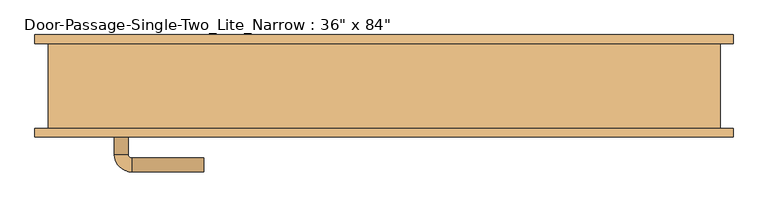
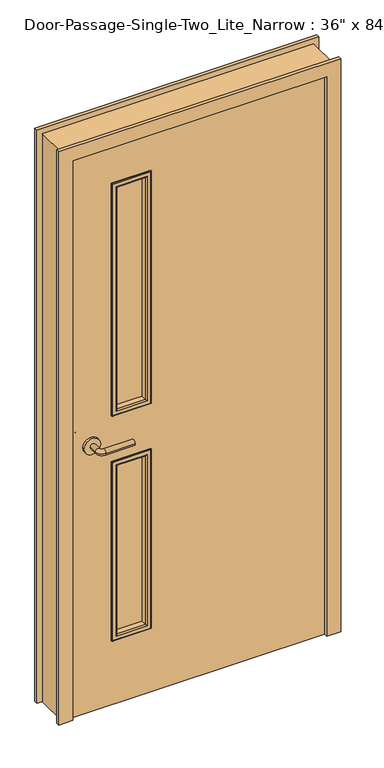
"""IFC4 building model written with IfcOpenShell, lengths in millimetres: door geometry."""

import ifcopenshell
import ifcopenshell.guid

model = None  # the IFC model being written
_history = None  # IfcOwnerHistory: only IFC2X3 demands one
_inside = {}  # id of a spatial element -> (the spatial element, [elements in it])
_under = {}  # id of a project, library or spatial element -> (it, [spatial elements below it])
_declared = {}  # id of a project -> (the project, [libraries it declares])
_typed = {}  # id of a type object -> (the type object, [elements of that type])
_made_of = {}  # id of a material, layer set ... -> (it, [elements and type objects made of it])


def new_model(schema):
    """Start an empty IFC model of exactly this schema.

    Asked for "IFC4X3", IfcOpenShell would pick the latest addendum, in which some entities
    have other attributes; the version numbers below select the first issue.
    IFC2X3 requires an IfcOwnerHistory on every rooted entity: one is made here for all.
    """
    global model, _history
    if schema == "IFC4X3":
        model = ifcopenshell.file(schema_version=(4, 3, 0, 0))
    else:
        model = ifcopenshell.file(schema=schema)
    _inside.clear()
    _under.clear()
    _declared.clear()
    _typed.clear()
    _made_of.clear()
    _history = None
    if model.schema == "IFC2X3":
        org = make("IfcOrganization", Name="unknown")
        user = make(
            "IfcPersonAndOrganization",
            ThePerson=make("IfcPerson", FamilyName="unknown"),
            TheOrganization=org,
        )
        app = make(
            "IfcApplication",
            ApplicationDeveloper=org,
            Version="unknown",
            ApplicationFullName="unknown",
            ApplicationIdentifier="unknown",
        )
        _history = make(
            "IfcOwnerHistory",
            OwningUser=user,
            OwningApplication=app,
            ChangeAction="ADDED",
            CreationDate=0,
        )
    return model


def make(cls, **values):
    """One entity of the class cls with the attributes given. An attribute that is None is left unset."""
    return model.create_entity(
        cls, **{name: value for name, value in values.items() if value is not None}
    )


def rooted(cls, **values):
    """An entity with a GlobalId (a new one), such as an element, a storey or a relation."""
    return make(cls, GlobalId=ifcopenshell.guid.new(), OwnerHistory=_history, **values)


def si_unit(unit_type, name, prefix=None):
    """IfcSIUnit, for example si_unit("LENGTHUNIT", "METRE", prefix="MILLI")."""
    return make("IfcSIUnit", UnitType=unit_type, Prefix=prefix, Name=name)


def assignment(units):
    """IfcUnitAssignment: the units of a project."""
    return None if units is None else make("IfcUnitAssignment", Units=units)


def point(xyz):
    """IfcCartesianPoint."""
    return None if xyz is None else make("IfcCartesianPoint", Coordinates=xyz)


def direction(xyz):
    """IfcDirection."""
    return None if xyz is None else make("IfcDirection", DirectionRatios=xyz)


def frame(location, z_axis=None, x_axis=None):
    """IfcAxis2Placement3D, a coordinate frame: its origin and axes. An axis left out is left unset."""
    return make(
        "IfcAxis2Placement3D",
        Location=point(location),
        Axis=direction(z_axis),
        RefDirection=direction(x_axis),
    )


def frame_2d(location, x_axis=None):
    """IfcAxis2Placement2D, a coordinate frame in the plane: its origin and x axis."""
    return make(
        "IfcAxis2Placement2D", Location=point(location), RefDirection=direction(x_axis)
    )


def origin():
    """The frame at (0, 0, 0) with its axes left unset."""
    return frame((0.0, 0.0, 0.0))


def place(relative_to, where):
    """IfcLocalPlacement: puts the frame where relative to a parent placement (None: the world)."""
    return make(
        "IfcLocalPlacement", PlacementRelTo=relative_to, RelativePlacement=where
    )


def context(
    kind, dimensions, precision=None, world=None, true_north=None, identifier=None
):
    """IfcGeometricRepresentationContext, for example the 3D "Model" context."""
    return make(
        "IfcGeometricRepresentationContext",
        ContextIdentifier=identifier,
        ContextType=kind,
        CoordinateSpaceDimension=dimensions,
        Precision=precision,
        WorldCoordinateSystem=world,
        TrueNorth=true_north,
    )


def project(units=None, contexts=None):
    """IfcProject with its units and contexts."""
    return rooted(
        "IfcProject",
        Name="project",
        RepresentationContexts=contexts,
        UnitsInContext=assignment(units),
    )


def spatial(cls, under=None, at=None, **own):
    """A site, building, storey or space (cls), placed at a placement, below another one or the project."""
    s = rooted(cls, ObjectPlacement=at, **own)
    if under is not None:
        _under.setdefault(under.id(), (under, []))[1].append(s)
    return s


def polyline(points):
    """IfcPolyline through the points."""
    return make("IfcPolyline", Points=[point(p) for p in points])


def circle_curve(where, radius):
    """IfcCircle in the frame where."""
    return make("IfcCircle", Position=where, Radius=radius)


def ellipse_curve(where, semi_axis1, semi_axis2):
    """IfcEllipse in the frame where."""
    return make(
        "IfcEllipse", Position=where, SemiAxis1=semi_axis1, SemiAxis2=semi_axis2
    )


def trimmed(basis, trim1, trim2, sense, master):
    """IfcTrimmedCurve: the piece of a basis curve between two trims."""
    return make(
        "IfcTrimmedCurve",
        BasisCurve=basis,
        Trim1=trim1,
        Trim2=trim2,
        SenseAgreement=sense,
        MasterRepresentation=master,
    )


def segment(curve, same_sense, transition):
    """IfcCompositeCurveSegment."""
    return make(
        "IfcCompositeCurveSegment",
        Transition=transition,
        SameSense=same_sense,
        ParentCurve=curve,
    )


def composite_curve(segments, self_intersect=None):
    """IfcCompositeCurve: segments joined end to end."""
    return make("IfcCompositeCurve", Segments=segments, SelfIntersect=self_intersect)


def outline(outer, holes=None, kind="AREA"):
    """IfcArbitraryClosedProfileDef: a profile drawn as a closed curve; with holes, ...WithVoids."""
    if holes is None:
        return make("IfcArbitraryClosedProfileDef", ProfileType=kind, OuterCurve=outer)
    return make(
        "IfcArbitraryProfileDefWithVoids",
        ProfileType=kind,
        OuterCurve=outer,
        InnerCurves=holes,
    )


def extrude(swept, where, along, depth):
    """IfcExtrudedAreaSolid: the profile swept, set in the frame where, extruded along a direction by depth."""
    return make(
        "IfcExtrudedAreaSolid",
        SweptArea=swept,
        Position=where,
        ExtrudedDirection=direction(along),
        Depth=depth,
    )


def faces_of(points, faces, orient=None, outer=None):
    """IfcFace entities. A face is a list of loops; a loop is a list of indices into points, from 0.

    orient and outer hold one flag for each loop. By default every Orientation is true, the
    first loop of a face is its IfcFaceOuterBound and the others are IfcFaceBound.
    """
    made = []
    for i, loops in enumerate(faces):
        bounds = []
        for j, loop in enumerate(loops):
            is_outer = j == 0 if outer is None else outer[i][j]
            bounds.append(
                make(
                    "IfcFaceOuterBound" if is_outer else "IfcFaceBound",
                    Bound=make("IfcPolyLoop", Polygon=[points[k] for k in loop]),
                    Orientation=True if orient is None else orient[i][j],
                )
            )
        made.append(make("IfcFace", Bounds=bounds))
    return made


def faceted_brep(points, faces, orient=None, outer=None, voids=None):
    """IfcFacetedBrep: a solid bounded by flat faces; with voids (closed shells), ...WithVoids."""
    shared = [point(p) for p in points]
    hull = make("IfcClosedShell", CfsFaces=faces_of(shared, faces, orient, outer))
    if voids is None:
        return make("IfcFacetedBrep", Outer=hull)
    return make(
        "IfcFacetedBrepWithVoids",
        Outer=hull,
        Voids=[
            make(cls, CfsFaces=faces_of(shared, fs, o, b)) for cls, fs, o, b in voids
        ],
    )


def shape(context_of_items, identifier, shape_type, items):
    """IfcShapeRepresentation: the items that make up one representation, for example the "Body"."""
    return make(
        "IfcShapeRepresentation",
        ContextOfItems=context_of_items,
        RepresentationIdentifier=identifier,
        RepresentationType=shape_type,
        Items=items,
    )


def source(mapping_origin, context_of_items, identifier, shape_type, items):
    """IfcRepresentationMap: a shape defined once, which mapped items show again and again."""
    return make(
        "IfcRepresentationMap",
        MappingOrigin=mapping_origin,
        MappedRepresentation=shape(context_of_items, identifier, shape_type, items),
    )


def transform(
    local_origin,
    x_axis=None,
    y_axis=None,
    z_axis=None,
    scale=None,
    scale2=None,
    scale3=None,
    uniform=True,
):
    """IfcCartesianTransformationOperator3D, or its non-uniform kind. x_axis, y_axis, z_axis: its Axis1, 2, 3."""
    if uniform:
        return make(
            "IfcCartesianTransformationOperator3D",
            Axis1=direction(x_axis),
            Axis2=direction(y_axis),
            LocalOrigin=point(local_origin),
            Scale=scale,
            Axis3=direction(z_axis),
        )
    return make(
        "IfcCartesianTransformationOperator3DnonUniform",
        Axis1=direction(x_axis),
        Axis2=direction(y_axis),
        LocalOrigin=point(local_origin),
        Scale=scale,
        Axis3=direction(z_axis),
        Scale2=scale2,
        Scale3=scale3,
    )


def mapped(mapping_source, mapping_target):
    """IfcMappedItem: shows the shape of a source again, moved by a transform."""
    return make(
        "IfcMappedItem", MappingSource=mapping_source, MappingTarget=mapping_target
    )


def made_of(thing, what):
    """Note that an element or type object is made of a material, layer set ...; save() writes the relation."""
    if what is not None:
        _made_of.setdefault(what.id(), (what, []))[1].append(thing)
    return thing


def element(
    cls,
    number,
    at=None,
    inside=None,
    cuts=None,
    type_object=None,
    material=None,
    context=None,
    identifier="Body",
    shape_type=None,
    held_by="IfcProductDefinitionShape",
    body=None,
    shapes=None,
    **own,
):
    """One element of the class cls, such as IfcWall. Its Tag is "e" and its number.

    at: its placement. inside: the storey or other place that contains it. cuts: it is an
    opening in that element (IfcRelVoidsElement). A single representation is given by context,
    identifier, shape_type and body (its items); several are given by shapes. held_by: the class
    of the entity that holds the representations. save() writes the other relations.
    """
    e = rooted(cls, Tag="e%d" % number, ObjectPlacement=at, **own)
    if body is not None:
        shapes = [shape(context, identifier, shape_type, body)]
    if shapes is not None:
        e.Representation = make(held_by, Representations=shapes)
    if inside is not None:
        _inside.setdefault(inside.id(), (inside, []))[1].append(e)
    if cuts is not None:
        rooted(
            "IfcRelVoidsElement", RelatingBuildingElement=cuts, RelatedOpeningElement=e
        )
    if type_object is not None:
        _typed.setdefault(type_object.id(), (type_object, []))[1].append(e)
    return made_of(e, material)


def aggregate(whole, parts):
    """IfcRelAggregates: a whole, such as a stair, and the parts it consists of."""
    return rooted("IfcRelAggregates", RelatingObject=whole, RelatedObjects=parts)


def save(model, path):
    """Write the relations noted so far, then the file.

    IfcRelAggregates (storeys below a building ...), IfcRelContainedInSpatialStructure (elements
    in a storey), IfcRelDefinesByType, IfcRelAssociatesMaterial and IfcRelDeclares: one each for
    every whole, place, type object, material and project.
    """
    for whole, parts in _under.values():
        aggregate(whole, parts)
    for where, things in _inside.values():
        rooted(
            "IfcRelContainedInSpatialStructure",
            RelatedElements=things,
            RelatingStructure=where,
        )
    for kind, things in _typed.values():
        rooted("IfcRelDefinesByType", RelatedObjects=things, RelatingType=kind)
    for what, things in _made_of.values():
        rooted("IfcRelAssociatesMaterial", RelatedObjects=things, RelatingMaterial=what)
    for by, libraries in _declared.values():
        rooted("IfcRelDeclares", RelatingContext=by, RelatedDefinitions=libraries)
    model.write(path)


def plane_surface(at):
    """IfcPlane: the flat surface through the origin of the frame at, square to its z axis."""
    return make("IfcPlane", Position=at)


def cylinder_surface(at, radius):
    """IfcCylindricalSurface: all points at the distance radius from the z axis of the frame at."""
    return make("IfcCylindricalSurface", Position=at, Radius=radius)


def revolved_surface(curve, axis_point, axis_direction):
    """IfcSurfaceOfRevolution: the curve turned about the line through axis_point along axis_direction."""
    return make(
        "IfcSurfaceOfRevolution",
        SweptCurve=make("IfcArbitraryOpenProfileDef", ProfileType="CURVE", Curve=curve),
        AxisPosition=make("IfcAxis1Placement", Location=point(axis_point), Axis=direction(axis_direction)),
    )


def advanced_brep(points, edges, surfaces, faces):
    """IfcAdvancedBrep: a solid bounded by faces that lie on surfaces and meet in shared edges.

    An edge is (start, end): straight between two places in points (the first is 0);
    or (start, end, curve); or (start, end, curve, False) where it runs against its curve.
    A face is (place in surfaces, loops), or (place, loops, False) where it looks against
    its surface's normal. A loop lists edges by number (the first is 1), with a minus sign
    where the edge is run from its end to its start. The first loop is the outer one.
    """
    corners = [point(p) for p in points]
    vertices = [make("IfcVertexPoint", VertexGeometry=c) for c in corners]
    made = []
    for start, end, *more in edges:
        made.append(
            make(
                "IfcEdgeCurve",
                EdgeStart=vertices[start],
                EdgeEnd=vertices[end],
                EdgeGeometry=more[0] if more else make("IfcPolyline", Points=[corners[start], corners[end]]),
                SameSense=more[1] if len(more) > 1 else True,
            )
        )
    hull = []
    for where, loops, *sense in faces:
        bounds = []
        for j, loop in enumerate(loops):
            ring = [make("IfcOrientedEdge", EdgeElement=made[abs(k) - 1], Orientation=k > 0) for k in loop]
            bounds.append(
                make(
                    "IfcFaceOuterBound" if j == 0 else "IfcFaceBound",
                    Bound=make("IfcEdgeLoop", EdgeList=ring),
                    Orientation=True,
                )
            )
        hull.append(make("IfcAdvancedFace", Bounds=bounds, FaceSurface=surfaces[where], SameSense=sense[0] if sense else True))
    return make("IfcAdvancedBrep", Outer=make("IfcClosedShell", CfsFaces=hull))


def door_7eef6684(model_context):
    return source(origin(), model_context, "Body", "SolidModel", [
        advanced_brep(
        [(-392.190625, -15.8125, 1016.0), (-372.190625, -15.8125, 1016.0), (-392.190625, 14.1875, 1016.0), (-372.190625, 14.1875, 1016.0), (-367.190625, 19.1875, 1016.0), (-367.190625, 39.1875, 1016.0), (-262.190625, 39.1875, 1016.0), (-262.190625, 19.1875, 1016.0)],
        [
            (0, 1, circle_curve(frame((-382.190625, -15.8125, 1016.0), z_axis=(0.0, -1.0, 0.0), x_axis=(1.0, 0.0, 0.0)), 10.0)),
            (1, 0, circle_curve(frame((-382.190625, -15.8125, 1016.0), z_axis=(0.0, -1.0, 0.0), x_axis=(1.0, 0.0, 0.0)), 10.0)),
            (0, 2),
            (2, 3, circle_curve(frame((-382.190625, 14.1875, 1016.0), z_axis=(0.0, -1.0, 0.0), x_axis=(1.0, 0.0, 0.0)), 10.0)),
            (3, 1),
            (3, 2, circle_curve(frame((-382.190625, 14.1875, 1016.0), z_axis=(0.0, -1.0, 0.0), x_axis=(1.0, 0.0, 0.0)), 10.0)),
            (4, 3, circle_curve(frame((-367.190625, 14.1875, 1016.0), z_axis=(0.0, 0.0, 1.0), x_axis=(-1.0, 0.0, 0.0)), 5.0)),
            (2, 5, circle_curve(frame((-367.190625, 14.1875, 1016.0), z_axis=(0.0, 0.0, -1.0), x_axis=(-1.0, 0.0, 0.0)), 25.0)),
            (5, 4, circle_curve(frame((-367.190625, 29.1875, 1016.0), z_axis=(-1.0, 0.0, 0.0), x_axis=(0.0, -1.0, 0.0)), 10.0)),
            (4, 5, circle_curve(frame((-367.190625, 29.1875, 1016.0), z_axis=(-1.0, 0.0, 0.0), x_axis=(0.0, -1.0, 0.0)), 10.0)),
            (6, 7, circle_curve(frame((-262.190625, 29.1875, 1016.0), z_axis=(1.0, 0.0, 0.0), x_axis=(0.0, -1.0, 0.0)), 10.0)),
            (7, 6, circle_curve(frame((-262.190625, 29.1875, 1016.0), z_axis=(1.0, 0.0, 0.0), x_axis=(0.0, -1.0, 0.0)), 10.0)),
            (5, 6),
            (7, 4),
        ],
        [
            plane_surface(frame((-382.190625, -15.8125, 1016.0), z_axis=(0.0, -1.0, 0.0), x_axis=(0.0, 0.0, 1.0))),
            cylinder_surface(frame((-382.190625, -15.8125, 1016.0), z_axis=(0.0, -1.0, 0.0), x_axis=(1.0, 0.0, 0.0)), 10.0),
            revolved_surface(trimmed(ellipse_curve(frame((-382.190625, 14.1875, 1016.0), z_axis=(0.0, -1.0, 0.0), x_axis=(1.0, 0.0, 0.0)), 10.0, 10.0), [point((-392.190625, 14.1875, 1016.0))], [point((-372.190625, 14.1875, 1016.0))], True, "CARTESIAN"), (-367.190625, 14.1875, 1016.0), (0.0, 0.0, -1.0)),
            revolved_surface(trimmed(ellipse_curve(frame((-382.190625, 14.1875, 1016.0), z_axis=(0.0, -1.0, 0.0), x_axis=(1.0, 0.0, 0.0)), 10.0, 10.0), [point((-372.190625, 14.1875, 1016.0))], [point((-392.190625, 14.1875, 1016.0))], True, "CARTESIAN"), (-367.190625, 14.1875, 1016.0), (0.0, 0.0, -1.0)),
            plane_surface(frame((-262.190625, 29.1875, 1016.0), z_axis=(1.0, 0.0, 0.0), x_axis=(0.0, 0.0, 1.0))),
            cylinder_surface(frame((-367.190625, 29.1875, 1016.0), z_axis=(-1.0, 0.0, 0.0), x_axis=(0.0, -1.0, 0.0)), 10.0),
        ],
        [
            (0, [[1, 2]]),
            (1, [[-1, 3, 4, 5]]),
            (1, [[-2, -5, 6, -3]]),
            (2, [[7, -4, 8, 9]]),
            (3, [[-8, -6, -7, 10]]),
            (4, [[11, 12]]),
            (5, [[-9, 13, -12, 14]]),
            (5, [[-10, -14, -11, -13]]),
        ],
    ),
        extrude(outline(composite_curve([segment(trimmed(circle_curve(frame_2d((1016.0, -384.690625)), 30.0), [point((1016.0, -414.690625))], [point((1016.0, -354.690625))], False, "CARTESIAN"), True, "CONTINUOUS"), segment(trimmed(circle_curve(frame_2d((1016.0, -384.690625)), 30.0), [point((1016.0, -354.690625))], [point((1016.0, -414.690625))], False, "CARTESIAN"), True, "CONTINUOUS")], self_intersect=False)), frame((0.0, -23.8125, 0.0), z_axis=(0.0, 1.0, 0.0), x_axis=(0.0, 0.0, 1.0)), (0.0, 0.0, 1.0), 8.0),
        advanced_brep(
        [(-392.190625, -76.2625, 1016.0), (-372.190625, -76.2625, 1016.0), (-372.190625, -106.2625, 1016.0), (-392.190625, -106.2625, 1016.0), (-367.190625, -111.2625, 1016.0), (-367.190625, -131.2625, 1016.0), (-262.190625, -131.2625, 1016.0), (-262.190625, -111.2625, 1016.0)],
        [
            (0, 1, circle_curve(frame((-382.190625, -76.2625, 1016.0), z_axis=(0.0, 1.0, 0.0), x_axis=(1.0, 0.0, 0.0)), 10.0)),
            (1, 0, circle_curve(frame((-382.190625, -76.2625, 1016.0), z_axis=(0.0, 1.0, 0.0), x_axis=(1.0, 0.0, 0.0)), 10.0)),
            (1, 2),
            (2, 3, circle_curve(frame((-382.190625, -106.2625, 1016.0), z_axis=(0.0, 1.0, 0.0), x_axis=(1.0, 0.0, 0.0)), 10.0)),
            (3, 0),
            (3, 2, circle_curve(frame((-382.190625, -106.2625, 1016.0), z_axis=(0.0, 1.0, 0.0), x_axis=(1.0, 0.0, 0.0)), 10.0)),
            (4, 5, circle_curve(frame((-367.190625, -121.2625, 1016.0), z_axis=(-1.0, 0.0, 0.0), x_axis=(0.0, 1.0, 0.0)), 10.0)),
            (5, 3, circle_curve(frame((-367.190625, -106.2625, 1016.0), z_axis=(0.0, 0.0, -1.0), x_axis=(-1.0, 0.0, 0.0)), 25.0)),
            (2, 4, circle_curve(frame((-367.190625, -106.2625, 1016.0), z_axis=(0.0, 0.0, 1.0), x_axis=(-1.0, 0.0, 0.0)), 5.0)),
            (5, 4, circle_curve(frame((-367.190625, -121.2625, 1016.0), z_axis=(-1.0, 0.0, 0.0), x_axis=(0.0, 1.0, 0.0)), 10.0)),
            (6, 7, circle_curve(frame((-262.190625, -121.2625, 1016.0), z_axis=(1.0, 0.0, 0.0), x_axis=(0.0, 1.0, 0.0)), 10.0)),
            (7, 6, circle_curve(frame((-262.190625, -121.2625, 1016.0), z_axis=(1.0, 0.0, 0.0), x_axis=(0.0, 1.0, 0.0)), 10.0)),
            (4, 7),
            (6, 5),
        ],
        [
            plane_surface(frame((-382.190625, -76.2625, 1016.0), z_axis=(0.0, 1.0, 0.0), x_axis=(0.0, 0.0, 1.0))),
            cylinder_surface(frame((-382.190625, -76.2625, 1016.0), z_axis=(0.0, 1.0, 0.0), x_axis=(1.0, 0.0, 0.0)), 10.0),
            revolved_surface(trimmed(ellipse_curve(frame((-382.190625, -106.2625, 1016.0), z_axis=(0.0, -1.0, 0.0), x_axis=(1.0, 0.0, 0.0)), 10.0, 10.0), [point((-392.190625, -106.2625, 1016.0))], [point((-372.190625, -106.2625, 1016.0))], True, "CARTESIAN"), (-367.190625, -106.2625, 1016.0), (0.0, 0.0, -1.0)),
            revolved_surface(trimmed(ellipse_curve(frame((-382.190625, -106.2625, 1016.0), z_axis=(0.0, -1.0, 0.0), x_axis=(1.0, 0.0, 0.0)), 10.0, 10.0), [point((-372.190625, -106.2625, 1016.0))], [point((-392.190625, -106.2625, 1016.0))], True, "CARTESIAN"), (-367.190625, -106.2625, 1016.0), (0.0, 0.0, -1.0)),
            plane_surface(frame((-262.190625, -121.2625, 1016.0), z_axis=(1.0, 0.0, 0.0), x_axis=(0.0, 0.0, 1.0))),
            cylinder_surface(frame((-367.190625, -121.2625, 1016.0), z_axis=(-1.0, 0.0, 0.0), x_axis=(0.0, 1.0, 0.0)), 10.0),
        ],
        [
            (0, [[1, 2]]),
            (1, [[3, 4, 5, -2]]),
            (1, [[-5, 6, -3, -1]]),
            (2, [[7, 8, -4, 9]]),
            (3, [[10, -9, -6, -8]]),
            (4, [[11, 12]]),
            (5, [[13, -11, 14, -7]]),
            (5, [[-14, -12, -13, -10]]),
        ],
    ),
        extrude(outline(composite_curve([segment(trimmed(circle_curve(frame_2d((1016.0, -384.690625)), 30.0), [point((1016.0, -414.690625))], [point((1016.0, -354.690625))], False, "CARTESIAN"), True, "CONTINUOUS"), segment(trimmed(circle_curve(frame_2d((1016.0, -384.690625)), 30.0), [point((1016.0, -354.690625))], [point((1016.0, -414.690625))], False, "CARTESIAN"), True, "CONTINUOUS")], self_intersect=False)), frame((0.0, -76.2625, 0.0), z_axis=(0.0, 1.0, 0.0), x_axis=(0.0, 0.0, 1.0)), (0.0, 0.0, 1.0), 8.0),
        faceted_brep([(457.2, -80.9625, 0.0), (457.2, -19.05, 0.0), (441.325, -19.05, 0.0), (441.325, 19.05, 0.0), (457.2, 19.05, 0.0), (457.2, 68.2625, 0.0), (508.0, 68.2625, 0.0), (508.0, 55.5625, 0.0), (488.95, 55.5625, 0.0), (488.95, -68.2625, 0.0), (508.0, -68.2625, 0.0), (508.0, -80.9625, 0.0), (508.0, -80.9625, 2184.4), (-508.0, -80.9625, 2184.4), (-508.0, -80.9625, 0.0), (-457.2, -80.9625, 0.0), (-457.2, -80.9625, 2133.6), (457.2, -80.9625, 2133.6), (508.0, -68.2625, 2184.4), (488.95, -68.2625, 2165.35), (-488.95, -68.2625, 2165.35), (-488.95, -68.2625, 0.0), (-508.0, -68.2625, 0.0), (-508.0, -68.2625, 2184.4), (488.95, 55.5625, 2165.35), (508.0, 55.5625, 2184.4), (-508.0, 55.5625, 2184.4), (-508.0, 55.5625, 0.0), (-488.95, 55.5625, 0.0), (-488.95, 55.5625, 2165.35), (508.0, 68.2625, 2184.4), (457.2, 68.2625, 2133.6), (-457.2, 68.2625, 2133.6), (-457.2, 68.2625, 0.0), (-508.0, 68.2625, 0.0), (-508.0, 68.2625, 2184.4), (457.2, 19.05, 2133.6), (441.325, 19.05, 2117.725), (-441.325, 19.05, 2117.725), (-441.325, 19.05, 0.0), (-457.2, 19.05, 0.0), (-457.2, 19.05, 2133.6), (441.325, -19.05, 2117.725), (457.2, -19.05, 2133.6), (-457.2, -19.05, 2133.6), (-457.2, -19.05, 0.0), (-441.325, -19.05, 0.0), (-441.325, -19.05, 2117.725)], [[[0, 1, 2, 3, 4, 5, 6, 7, 8, 9, 10, 11]], [[11, 12, 13, 14, 15, 16, 17, 0]], [[10, 18, 12, 11]], [[9, 19, 20, 21, 22, 23, 18, 10]], [[8, 24, 19, 9]], [[7, 25, 26, 27, 28, 29, 24, 8]], [[6, 30, 25, 7]], [[5, 31, 32, 33, 34, 35, 30, 6]], [[4, 36, 31, 5]], [[3, 37, 38, 39, 40, 41, 36, 4]], [[2, 42, 37, 3]], [[1, 43, 44, 45, 46, 47, 42, 2]], [[0, 17, 43, 1]], [[18, 23, 13, 12]], [[24, 29, 20, 19]], [[30, 35, 26, 25]], [[36, 41, 32, 31]], [[42, 47, 38, 37]], [[17, 16, 44, 43]], [[15, 14, 22, 21, 28, 27, 34, 33, 40, 39, 46, 45]], [[23, 22, 14, 13]], [[29, 28, 21, 20]], [[35, 34, 27, 26]], [[41, 40, 33, 32]], [[47, 46, 39, 38]], [[16, 15, 45, 44]]]),
        extrude(outline(polyline([(2133.6, -457.2), (0.0, -457.2), (0.0, 457.2), (2133.6, 457.2), (2133.6, -457.2)]), holes=[polyline([(1981.2, -304.8), (1981.2, -177.8), (1111.25, -177.8), (1111.25, -304.8), (1981.2, -304.8)]), polyline([(920.75, -304.8), (920.75, -177.8), (254.0, -177.8), (254.0, -304.8), (920.75, -304.8)])]), frame((0.0, -68.2625, 0.0), z_axis=(0.0, 1.0, 0.0), x_axis=(0.0, 0.0, 1.0)), (0.0, 0.0, 1.0), 44.45),
        extrude(outline(polyline([(-177.8, -42.8625), (-177.8, -49.2125), (-304.8, -49.2125), (-304.8, -42.8625), (-177.8, -42.8625)])), frame((0.0, 0.0, 1111.25), z_axis=(0.0, 0.0, 1.0), x_axis=(1.0, 0.0, 0.0)), (0.0, 0.0, 1.0), 869.95),
        extrude(outline(polyline([(-177.8, -42.8625), (-177.8, -49.2125), (-304.8, -49.2125), (-304.8, -42.8625), (-177.8, -42.8625)])), frame((0.0, 0.0, 254.0), z_axis=(0.0, 0.0, 1.0), x_axis=(1.0, 0.0, 0.0)), (0.0, 0.0, 1.0), 666.75),
        advanced_brep(
        [(-177.8, -42.8625, 920.75), (-177.8, -42.8625, 254.0), (-177.8, -23.8125, 254.0), (-177.8, -23.8125, 920.75), (-189.8, -22.8125, 908.75), (-189.8, -22.8125, 266.0), (-189.8, -42.8625, 266.0), (-189.8, -42.8625, 908.75), (-184.8, -17.8125, 913.75), (-184.8, -17.8125, 261.0), (-169.8, -19.8125, 928.75), (-169.8, -19.8125, 246.0), (-171.8, -17.8125, 248.0), (-171.8, -17.8125, 926.75), (-169.8, -23.8125, 928.75), (-169.8, -23.8125, 246.0), (-304.8, -42.8625, 254.0), (-304.8, -23.8125, 254.0), (-292.8, -22.8125, 266.0), (-292.8, -42.8625, 266.0), (-297.8, -17.8125, 261.0), (-312.8, -19.8125, 246.0), (-310.8, -17.8125, 248.0), (-312.8, -23.8125, 246.0), (-304.8, -42.8625, 920.75), (-304.8, -23.8125, 920.75), (-292.8, -22.8125, 908.75), (-292.8, -42.8625, 908.75), (-297.8, -17.8125, 913.75), (-312.8, -19.8125, 928.75), (-310.8, -17.8125, 926.75), (-312.8, -23.8125, 928.75)],
        [
            (0, 1),
            (1, 2),
            (2, 3),
            (3, 0),
            (4, 5),
            (5, 6),
            (6, 7),
            (7, 4),
            (8, 9),
            (9, 5, ellipse_curve(frame((-184.8, -22.8125, 261.0), z_axis=(0.7071067811865475, 0.0, 0.7071067811865475), x_axis=(-0.7071067811865474, 0.0, 0.7071067811865476)), 7.0710678, 5.0)),
            (4, 8, ellipse_curve(frame((-184.8, -22.8125, 913.75), z_axis=(0.7071067811865475, 0.0, -0.7071067811865475), x_axis=(0.7071067811865474, 0.0, 0.7071067811865476)), 7.0710678, 5.0)),
            (10, 11),
            (11, 12, ellipse_curve(frame((-171.8, -19.8125, 248.0), z_axis=(0.7071067811865475, 0.0, 0.7071067811865475), x_axis=(-0.7071067811865474, 0.0, 0.7071067811865476)), 2.8284271, 2.0)),
            (12, 13),
            (13, 10, ellipse_curve(frame((-171.8, -19.8125, 926.75), z_axis=(0.7071067811865475, 0.0, -0.7071067811865475), x_axis=(0.7071067811865474, 0.0, 0.7071067811865476)), 2.8284271, 2.0)),
            (14, 15),
            (15, 11),
            (10, 14),
            (1, 16),
            (16, 17),
            (17, 2),
            (5, 18),
            (18, 19),
            (19, 6),
            (9, 20),
            (20, 18, ellipse_curve(frame((-297.8, -22.8125, 261.0), z_axis=(0.7071067811865475, 0.0, -0.7071067811865475), x_axis=(0.7071067811865476, 0.0, 0.7071067811865474)), 7.0710678, 5.0)),
            (11, 21),
            (21, 22, ellipse_curve(frame((-310.8, -19.8125, 248.0), z_axis=(0.7071067811865475, 0.0, -0.7071067811865475), x_axis=(0.7071067811865476, 0.0, 0.7071067811865474)), 2.8284271, 2.0)),
            (22, 12),
            (15, 23),
            (23, 21),
            (16, 24),
            (24, 25),
            (25, 17),
            (18, 26),
            (26, 27),
            (27, 19),
            (20, 28),
            (28, 26, ellipse_curve(frame((-297.8, -22.8125, 913.75), z_axis=(-0.7071067811865475, 0.0, -0.7071067811865475), x_axis=(0.7071067811865474, 0.0, -0.7071067811865476)), 7.0710678, 5.0)),
            (21, 29),
            (29, 30, ellipse_curve(frame((-310.8, -19.8125, 926.75), z_axis=(-0.7071067811865475, 0.0, -0.7071067811865475), x_axis=(0.7071067811865474, 0.0, -0.7071067811865476)), 2.8284271, 2.0)),
            (30, 22),
            (23, 31),
            (31, 29),
            (14, 31),
            (25, 3),
            (24, 0),
            (27, 7),
            (26, 4),
            (28, 8),
            (30, 13),
            (29, 10),
        ],
        [
            plane_surface(frame((-177.8, -23.8125, 920.75), z_axis=(1.0, 0.0, 0.0), x_axis=(0.0, 0.0, -1.0))),
            plane_surface(frame((-189.8, -42.8625, 908.75), z_axis=(-1.0, 0.0, 0.0), x_axis=(0.0, 0.0, -1.0))),
            cylinder_surface(frame((-184.8, -22.8125, 920.75), z_axis=(0.0, 0.0, 1.0), x_axis=(1.0, 0.0, 0.0)), 5.0),
            cylinder_surface(frame((-171.8, -19.8125, 920.75), z_axis=(0.0, 0.0, 1.0), x_axis=(1.0, 0.0, 0.0)), 2.0),
            plane_surface(frame((-169.8, -19.8125, 928.75), z_axis=(1.0, 0.0, 0.0), x_axis=(0.0, 0.0, -1.0))),
            plane_surface(frame((-177.8, -23.8125, 254.0), z_axis=(0.0, 0.0, -1.0), x_axis=(-1.0, 0.0, 0.0))),
            plane_surface(frame((-189.8, -42.8625, 266.0), z_axis=(0.0, 0.0, 1.0), x_axis=(-1.0, 0.0, 0.0))),
            cylinder_surface(frame((-177.8, -22.8125, 261.0), z_axis=(1.0, 0.0, 0.0), x_axis=(0.0, 0.0, -1.0)), 5.0),
            cylinder_surface(frame((-177.8, -19.8125, 248.0), z_axis=(1.0, 0.0, 0.0), x_axis=(0.0, 0.0, -1.0)), 2.0),
            plane_surface(frame((-169.8, -19.8125, 246.0), z_axis=(0.0, 0.0, -1.0), x_axis=(-1.0, 0.0, 0.0))),
            plane_surface(frame((-304.8, -23.8125, 254.0), z_axis=(-1.0, 0.0, 0.0), x_axis=(0.0, 0.0, 1.0))),
            plane_surface(frame((-292.8, -42.8625, 266.0), z_axis=(1.0, 0.0, 0.0), x_axis=(0.0, 0.0, 1.0))),
            cylinder_surface(frame((-297.8, -22.8125, 254.0), z_axis=(0.0, 0.0, -1.0), x_axis=(-1.0, 0.0, 0.0)), 5.0),
            cylinder_surface(frame((-310.8, -19.8125, 254.0), z_axis=(0.0, 0.0, -1.0), x_axis=(-1.0, 0.0, 0.0)), 2.0),
            plane_surface(frame((-312.8, -19.8125, 246.0), z_axis=(-1.0, 0.0, 0.0), x_axis=(0.0, 0.0, 1.0))),
            plane_surface(frame((-312.8, -23.8125, 928.75), z_axis=(0.0, -1.0, 0.0), x_axis=(1.0, 0.0, 0.0))),
            plane_surface(frame((-304.8, -23.8125, 920.75), z_axis=(0.0, 0.0, 1.0), x_axis=(1.0, 0.0, 0.0))),
            plane_surface(frame((-304.8, -42.8625, 920.75), z_axis=(0.0, -1.0, 0.0), x_axis=(1.0, 0.0, 0.0))),
            plane_surface(frame((-292.8, -42.8625, 908.75), z_axis=(0.0, 0.0, -1.0), x_axis=(1.0, 0.0, 0.0))),
            cylinder_surface(frame((-304.8, -22.8125, 913.75), z_axis=(-1.0, 0.0, 0.0), x_axis=(0.0, 0.0, 1.0)), 5.0),
            plane_surface(frame((-297.8, -17.8125, 913.75), z_axis=(0.0, 1.0, 0.0), x_axis=(1.0, 0.0, 0.0))),
            cylinder_surface(frame((-304.8, -19.8125, 926.75), z_axis=(-1.0, 0.0, 0.0), x_axis=(0.0, 0.0, 1.0)), 2.0),
            plane_surface(frame((-312.8, -19.8125, 928.75), z_axis=(0.0, 0.0, 1.0), x_axis=(1.0, 0.0, 0.0))),
        ],
        [
            (0, [[1, 2, 3, 4]]),
            (1, [[5, 6, 7, 8]]),
            (2, [[9, 10, -5, 11]]),
            (3, [[12, 13, 14, 15]]),
            (4, [[16, 17, -12, 18]]),
            (5, [[19, 20, 21, -2]]),
            (6, [[22, 23, 24, -6]]),
            (7, [[25, 26, -22, -10]]),
            (8, [[27, 28, 29, -13]]),
            (9, [[30, 31, -27, -17]]),
            (10, [[32, 33, 34, -20]]),
            (11, [[35, 36, 37, -23]]),
            (12, [[38, 39, -35, -26]]),
            (13, [[40, 41, 42, -28]]),
            (14, [[43, 44, -40, -31]]),
            (15, [[-16, 45, -43, -30], [-3, -21, -34, 46]]),
            (16, [[47, -4, -46, -33]]),
            (17, [[-1, -47, -32, -19], [-7, -24, -37, 48]]),
            (18, [[49, -8, -48, -36]]),
            (19, [[50, -11, -49, -39]]),
            (20, [[-14, -29, -42, 51], [-9, -50, -38, -25]]),
            (21, [[52, -15, -51, -41]]),
            (22, [[-45, -18, -52, -44]]),
        ],
    ),
        advanced_brep(
        [(-304.8, -49.2125, 920.75), (-304.8, -49.2125, 254.0), (-304.8, -68.2625, 254.0), (-304.8, -68.2625, 920.75), (-292.8, -69.2625, 908.75), (-292.8, -69.2625, 266.0), (-292.8, -49.2125, 266.0), (-292.8, -49.2125, 908.75), (-297.8, -74.2625, 913.75), (-297.8, -74.2625, 261.0), (-312.8, -72.2625, 928.75), (-312.8, -72.2625, 246.0), (-310.8, -74.2625, 248.0), (-310.8, -74.2625, 926.75), (-312.8, -68.2625, 928.75), (-312.8, -68.2625, 246.0), (-177.8, -49.2125, 254.0), (-177.8, -68.2625, 254.0), (-189.8, -69.2625, 266.0), (-189.8, -49.2125, 266.0), (-184.8, -74.2625, 261.0), (-169.8, -72.2625, 246.0), (-171.8, -74.2625, 248.0), (-169.8, -68.2625, 246.0), (-177.8, -49.2125, 920.75), (-177.8, -68.2625, 920.75), (-189.8, -69.2625, 908.75), (-189.8, -49.2125, 908.75), (-184.8, -74.2625, 913.75), (-169.8, -72.2625, 928.75), (-171.8, -74.2625, 926.75), (-169.8, -68.2625, 928.75)],
        [
            (0, 1),
            (1, 2),
            (2, 3),
            (3, 0),
            (4, 5),
            (5, 6),
            (6, 7),
            (7, 4),
            (8, 9),
            (9, 5, ellipse_curve(frame((-297.8, -69.2625, 261.0), z_axis=(-0.7071067811865475, 0.0, 0.7071067811865475), x_axis=(0.7071067811865474, 0.0, 0.7071067811865476)), 7.0710678, 5.0)),
            (4, 8, ellipse_curve(frame((-297.8, -69.2625, 913.75), z_axis=(-0.7071067811865475, 0.0, -0.7071067811865475), x_axis=(-0.7071067811865474, 0.0, 0.7071067811865476)), 7.0710678, 5.0)),
            (10, 11),
            (11, 12, ellipse_curve(frame((-310.8, -72.2625, 248.0), z_axis=(-0.7071067811865475, 0.0, 0.7071067811865475), x_axis=(0.7071067811865474, 0.0, 0.7071067811865476)), 2.8284271, 2.0)),
            (12, 13),
            (13, 10, ellipse_curve(frame((-310.8, -72.2625, 926.75), z_axis=(-0.7071067811865475, 0.0, -0.7071067811865475), x_axis=(-0.7071067811865474, 0.0, 0.7071067811865476)), 2.8284271, 2.0)),
            (14, 15),
            (15, 11),
            (10, 14),
            (1, 16),
            (16, 17),
            (17, 2),
            (5, 18),
            (18, 19),
            (19, 6),
            (9, 20),
            (20, 18, ellipse_curve(frame((-184.8, -69.2625, 261.0), z_axis=(-0.7071067811865475, 0.0, -0.7071067811865475), x_axis=(-0.7071067811865476, 0.0, 0.7071067811865474)), 7.0710678, 5.0)),
            (11, 21),
            (21, 22, ellipse_curve(frame((-171.8, -72.2625, 248.0), z_axis=(-0.7071067811865475, 0.0, -0.7071067811865475), x_axis=(-0.7071067811865476, 0.0, 0.7071067811865474)), 2.8284271, 2.0)),
            (22, 12),
            (15, 23),
            (23, 21),
            (16, 24),
            (24, 25),
            (25, 17),
            (18, 26),
            (26, 27),
            (27, 19),
            (20, 28),
            (28, 26, ellipse_curve(frame((-184.8, -69.2625, 913.75), z_axis=(0.7071067811865475, 0.0, -0.7071067811865475), x_axis=(-0.7071067811865474, 0.0, -0.7071067811865476)), 7.0710678, 5.0)),
            (21, 29),
            (29, 30, ellipse_curve(frame((-171.8, -72.2625, 926.75), z_axis=(0.7071067811865475, 0.0, -0.7071067811865475), x_axis=(-0.7071067811865474, 0.0, -0.7071067811865476)), 2.8284271, 2.0)),
            (30, 22),
            (23, 31),
            (31, 29),
            (14, 31),
            (25, 3),
            (24, 0),
            (27, 7),
            (26, 4),
            (28, 8),
            (30, 13),
            (29, 10),
        ],
        [
            plane_surface(frame((-304.8, -68.2625, 920.75), z_axis=(-1.0, 0.0, 0.0), x_axis=(0.0, 0.0, -1.0))),
            plane_surface(frame((-292.8, -49.2125, 908.75), z_axis=(1.0, 0.0, 0.0), x_axis=(0.0, 0.0, -1.0))),
            cylinder_surface(frame((-297.8, -69.2625, 920.75), z_axis=(0.0, 0.0, 1.0), x_axis=(-1.0, 0.0, 0.0)), 5.0),
            cylinder_surface(frame((-310.8, -72.2625, 920.75), z_axis=(0.0, 0.0, 1.0), x_axis=(-1.0, 0.0, 0.0)), 2.0),
            plane_surface(frame((-312.8, -72.2625, 928.75), z_axis=(-1.0, 0.0, 0.0), x_axis=(0.0, 0.0, -1.0))),
            plane_surface(frame((-304.8, -68.2625, 254.0), z_axis=(0.0, 0.0, -1.0), x_axis=(1.0, 0.0, 0.0))),
            plane_surface(frame((-292.8, -49.2125, 266.0), z_axis=(0.0, 0.0, 1.0), x_axis=(1.0, 0.0, 0.0))),
            cylinder_surface(frame((-304.8, -69.2625, 261.0), z_axis=(-1.0, 0.0, 0.0), x_axis=(0.0, 0.0, -1.0)), 5.0),
            cylinder_surface(frame((-304.8, -72.2625, 248.0), z_axis=(-1.0, 0.0, 0.0), x_axis=(0.0, 0.0, -1.0)), 2.0),
            plane_surface(frame((-312.8, -72.2625, 246.0), z_axis=(0.0, 0.0, -1.0), x_axis=(1.0, 0.0, 0.0))),
            plane_surface(frame((-177.8, -68.2625, 254.0), z_axis=(1.0, 0.0, 0.0), x_axis=(0.0, 0.0, 1.0))),
            plane_surface(frame((-189.8, -49.2125, 266.0), z_axis=(-1.0, 0.0, 0.0), x_axis=(0.0, 0.0, 1.0))),
            cylinder_surface(frame((-184.8, -69.2625, 254.0), z_axis=(0.0, 0.0, -1.0), x_axis=(1.0, 0.0, 0.0)), 5.0),
            cylinder_surface(frame((-171.8, -72.2625, 254.0), z_axis=(0.0, 0.0, -1.0), x_axis=(1.0, 0.0, 0.0)), 2.0),
            plane_surface(frame((-169.8, -72.2625, 246.0), z_axis=(1.0, 0.0, 0.0), x_axis=(0.0, 0.0, 1.0))),
            plane_surface(frame((-169.8, -68.2625, 928.75), z_axis=(0.0, 1.0, 0.0), x_axis=(-1.0, 0.0, 0.0))),
            plane_surface(frame((-177.8, -68.2625, 920.75), z_axis=(0.0, 0.0, 1.0), x_axis=(-1.0, 0.0, 0.0))),
            plane_surface(frame((-177.8, -49.2125, 920.75), z_axis=(0.0, 1.0, 0.0), x_axis=(-1.0, 0.0, 0.0))),
            plane_surface(frame((-189.8, -49.2125, 908.75), z_axis=(0.0, 0.0, -1.0), x_axis=(-1.0, 0.0, 0.0))),
            cylinder_surface(frame((-177.8, -69.2625, 913.75), z_axis=(1.0, 0.0, 0.0), x_axis=(0.0, 0.0, 1.0)), 5.0),
            plane_surface(frame((-184.8, -74.2625, 913.75), z_axis=(0.0, -1.0, 0.0), x_axis=(-1.0, 0.0, 0.0))),
            cylinder_surface(frame((-177.8, -72.2625, 926.75), z_axis=(1.0, 0.0, 0.0), x_axis=(0.0, 0.0, 1.0)), 2.0),
            plane_surface(frame((-169.8, -72.2625, 928.75), z_axis=(0.0, 0.0, 1.0), x_axis=(-1.0, 0.0, 0.0))),
        ],
        [
            (0, [[1, 2, 3, 4]]),
            (1, [[5, 6, 7, 8]]),
            (2, [[9, 10, -5, 11]]),
            (3, [[12, 13, 14, 15]]),
            (4, [[16, 17, -12, 18]]),
            (5, [[19, 20, 21, -2]]),
            (6, [[22, 23, 24, -6]]),
            (7, [[25, 26, -22, -10]]),
            (8, [[27, 28, 29, -13]]),
            (9, [[30, 31, -27, -17]]),
            (10, [[32, 33, 34, -20]]),
            (11, [[35, 36, 37, -23]]),
            (12, [[38, 39, -35, -26]]),
            (13, [[40, 41, 42, -28]]),
            (14, [[43, 44, -40, -31]]),
            (15, [[-16, 45, -43, -30], [-3, -21, -34, 46]]),
            (16, [[47, -4, -46, -33]]),
            (17, [[-1, -47, -32, -19], [-7, -24, -37, 48]]),
            (18, [[49, -8, -48, -36]]),
            (19, [[50, -11, -49, -39]]),
            (20, [[-14, -29, -42, 51], [-9, -50, -38, -25]]),
            (21, [[52, -15, -51, -41]]),
            (22, [[-45, -18, -52, -44]]),
        ],
    ),
        advanced_brep(
        [(-304.8, -42.8625, 1111.25), (-304.8, -42.8625, 1981.2), (-304.8, -23.8125, 1981.2), (-304.8, -23.8125, 1111.25), (-292.8, -22.8125, 1123.25), (-292.8, -22.8125, 1969.2), (-292.8, -42.8625, 1969.2), (-292.8, -42.8625, 1123.25), (-297.8, -17.8125, 1118.25), (-297.8, -17.8125, 1974.2), (-312.8, -19.8125, 1103.25), (-312.8, -19.8125, 1989.2), (-310.8, -17.8125, 1987.2), (-310.8, -17.8125, 1105.25), (-312.8, -23.8125, 1103.25), (-312.8, -23.8125, 1989.2), (-177.8, -42.8625, 1981.2), (-177.8, -23.8125, 1981.2), (-189.8, -22.8125, 1969.2), (-189.8, -42.8625, 1969.2), (-184.8, -17.8125, 1974.2), (-169.8, -19.8125, 1989.2), (-171.8, -17.8125, 1987.2), (-169.8, -23.8125, 1989.2), (-177.8, -42.8625, 1111.25), (-177.8, -23.8125, 1111.25), (-189.8, -22.8125, 1123.25), (-189.8, -42.8625, 1123.25), (-184.8, -17.8125, 1118.25), (-169.8, -19.8125, 1103.25), (-171.8, -17.8125, 1105.25), (-169.8, -23.8125, 1103.25)],
        [
            (0, 1),
            (1, 2),
            (2, 3),
            (3, 0),
            (4, 5),
            (5, 6),
            (6, 7),
            (7, 4),
            (8, 9),
            (9, 5, ellipse_curve(frame((-297.8, -22.8125, 1974.2), z_axis=(-0.7071067811865475, 0.0, -0.7071067811865475), x_axis=(0.7071067811865474, 0.0, -0.7071067811865476)), 7.0710678, 5.0)),
            (4, 8, ellipse_curve(frame((-297.8, -22.8125, 1118.25), z_axis=(-0.7071067811865475, 0.0, 0.7071067811865475), x_axis=(-0.7071067811865474, 0.0, -0.7071067811865476)), 7.0710678, 5.0)),
            (10, 11),
            (11, 12, ellipse_curve(frame((-310.8, -19.8125, 1987.2), z_axis=(-0.7071067811865475, 0.0, -0.7071067811865475), x_axis=(0.7071067811865474, 0.0, -0.7071067811865476)), 2.8284271, 2.0)),
            (12, 13),
            (13, 10, ellipse_curve(frame((-310.8, -19.8125, 1105.25), z_axis=(-0.7071067811865475, 0.0, 0.7071067811865475), x_axis=(-0.7071067811865474, 0.0, -0.7071067811865476)), 2.8284271, 2.0)),
            (14, 15),
            (15, 11),
            (10, 14),
            (1, 16),
            (16, 17),
            (17, 2),
            (5, 18),
            (18, 19),
            (19, 6),
            (9, 20),
            (20, 18, ellipse_curve(frame((-184.8, -22.8125, 1974.2), z_axis=(-0.7071067811865475, 0.0, 0.7071067811865475), x_axis=(-0.7071067811865476, 0.0, -0.7071067811865474)), 7.0710678, 5.0)),
            (11, 21),
            (21, 22, ellipse_curve(frame((-171.8, -19.8125, 1987.2), z_axis=(-0.7071067811865475, 0.0, 0.7071067811865475), x_axis=(-0.7071067811865476, 0.0, -0.7071067811865474)), 2.8284271, 2.0)),
            (22, 12),
            (15, 23),
            (23, 21),
            (16, 24),
            (24, 25),
            (25, 17),
            (18, 26),
            (26, 27),
            (27, 19),
            (20, 28),
            (28, 26, ellipse_curve(frame((-184.8, -22.8125, 1118.25), z_axis=(0.7071067811865475, 0.0, 0.7071067811865475), x_axis=(-0.7071067811865474, 0.0, 0.7071067811865476)), 7.0710678, 5.0)),
            (21, 29),
            (29, 30, ellipse_curve(frame((-171.8, -19.8125, 1105.25), z_axis=(0.7071067811865475, 0.0, 0.7071067811865475), x_axis=(-0.7071067811865474, 0.0, 0.7071067811865476)), 2.8284271, 2.0)),
            (30, 22),
            (23, 31),
            (31, 29),
            (14, 31),
            (25, 3),
            (24, 0),
            (27, 7),
            (26, 4),
            (28, 8),
            (30, 13),
            (29, 10),
        ],
        [
            plane_surface(frame((-304.8, -23.8125, 1111.25), z_axis=(-1.0, 0.0, 0.0), x_axis=(0.0, 0.0, 1.0))),
            plane_surface(frame((-292.8, -42.8625, 1123.25), z_axis=(1.0, 0.0, 0.0), x_axis=(0.0, 0.0, 1.0))),
            cylinder_surface(frame((-297.8, -22.8125, 1111.25), z_axis=(0.0, 0.0, -1.0), x_axis=(-1.0, 0.0, 0.0)), 5.0),
            cylinder_surface(frame((-310.8, -19.8125, 1111.25), z_axis=(0.0, 0.0, -1.0), x_axis=(-1.0, 0.0, 0.0)), 2.0),
            plane_surface(frame((-312.8, -19.8125, 1103.25), z_axis=(-1.0, 0.0, 0.0), x_axis=(0.0, 0.0, 1.0))),
            plane_surface(frame((-304.8, -23.8125, 1981.2), z_axis=(0.0, 0.0, 1.0), x_axis=(1.0, 0.0, 0.0))),
            plane_surface(frame((-292.8, -42.8625, 1969.2), z_axis=(0.0, 0.0, -1.0), x_axis=(1.0, 0.0, 0.0))),
            cylinder_surface(frame((-304.8, -22.8125, 1974.2), z_axis=(-1.0, 0.0, 0.0), x_axis=(0.0, 0.0, 1.0)), 5.0),
            cylinder_surface(frame((-304.8, -19.8125, 1987.2), z_axis=(-1.0, 0.0, 0.0), x_axis=(0.0, 0.0, 1.0)), 2.0),
            plane_surface(frame((-312.8, -19.8125, 1989.2), z_axis=(0.0, 0.0, 1.0), x_axis=(1.0, 0.0, 0.0))),
            plane_surface(frame((-177.8, -23.8125, 1981.2), z_axis=(1.0, 0.0, 0.0), x_axis=(0.0, 0.0, -1.0))),
            plane_surface(frame((-189.8, -42.8625, 1969.2), z_axis=(-1.0, 0.0, 0.0), x_axis=(0.0, 0.0, -1.0))),
            cylinder_surface(frame((-184.8, -22.8125, 1981.2), z_axis=(0.0, 0.0, 1.0), x_axis=(1.0, 0.0, 0.0)), 5.0),
            cylinder_surface(frame((-171.8, -19.8125, 1981.2), z_axis=(0.0, 0.0, 1.0), x_axis=(1.0, 0.0, 0.0)), 2.0),
            plane_surface(frame((-169.8, -19.8125, 1989.2), z_axis=(1.0, 0.0, 0.0), x_axis=(0.0, 0.0, -1.0))),
            plane_surface(frame((-169.8, -23.8125, 1103.25), z_axis=(0.0, -1.0, 0.0), x_axis=(-1.0, 0.0, 0.0))),
            plane_surface(frame((-177.8, -23.8125, 1111.25), z_axis=(0.0, 0.0, -1.0), x_axis=(-1.0, 0.0, 0.0))),
            plane_surface(frame((-177.8, -42.8625, 1111.25), z_axis=(0.0, -1.0, 0.0), x_axis=(-1.0, 0.0, 0.0))),
            plane_surface(frame((-189.8, -42.8625, 1123.25), z_axis=(0.0, 0.0, 1.0), x_axis=(-1.0, 0.0, 0.0))),
            cylinder_surface(frame((-177.8, -22.8125, 1118.25), z_axis=(1.0, 0.0, 0.0), x_axis=(0.0, 0.0, -1.0)), 5.0),
            plane_surface(frame((-184.8, -17.8125, 1118.25), z_axis=(0.0, 1.0, 0.0), x_axis=(-1.0, 0.0, 0.0))),
            cylinder_surface(frame((-177.8, -19.8125, 1105.25), z_axis=(1.0, 0.0, 0.0), x_axis=(0.0, 0.0, -1.0)), 2.0),
            plane_surface(frame((-169.8, -19.8125, 1103.25), z_axis=(0.0, 0.0, -1.0), x_axis=(-1.0, 0.0, 0.0))),
        ],
        [
            (0, [[1, 2, 3, 4]]),
            (1, [[5, 6, 7, 8]]),
            (2, [[9, 10, -5, 11]]),
            (3, [[12, 13, 14, 15]]),
            (4, [[16, 17, -12, 18]]),
            (5, [[19, 20, 21, -2]]),
            (6, [[22, 23, 24, -6]]),
            (7, [[25, 26, -22, -10]]),
            (8, [[27, 28, 29, -13]]),
            (9, [[30, 31, -27, -17]]),
            (10, [[32, 33, 34, -20]]),
            (11, [[35, 36, 37, -23]]),
            (12, [[38, 39, -35, -26]]),
            (13, [[40, 41, 42, -28]]),
            (14, [[43, 44, -40, -31]]),
            (15, [[-16, 45, -43, -30], [-3, -21, -34, 46]]),
            (16, [[47, -4, -46, -33]]),
            (17, [[-1, -47, -32, -19], [-7, -24, -37, 48]]),
            (18, [[49, -8, -48, -36]]),
            (19, [[50, -11, -49, -39]]),
            (20, [[-14, -29, -42, 51], [-9, -50, -38, -25]]),
            (21, [[52, -15, -51, -41]]),
            (22, [[-45, -18, -52, -44]]),
        ],
    ),
        advanced_brep(
        [(-304.8, -49.2125, 1981.2), (-304.8, -49.2125, 1111.25), (-304.8, -68.2625, 1111.25), (-304.8, -68.2625, 1981.2), (-292.8, -69.2625, 1969.2), (-292.8, -69.2625, 1123.25), (-292.8, -49.2125, 1123.25), (-292.8, -49.2125, 1969.2), (-297.8, -74.2625, 1974.2), (-297.8, -74.2625, 1118.25), (-312.8, -72.2625, 1989.2), (-312.8, -72.2625, 1103.25), (-310.8, -74.2625, 1105.25), (-310.8, -74.2625, 1987.2), (-312.8, -68.2625, 1989.2), (-312.8, -68.2625, 1103.25), (-177.8, -49.2125, 1111.25), (-177.8, -68.2625, 1111.25), (-189.8, -69.2625, 1123.25), (-189.8, -49.2125, 1123.25), (-184.8, -74.2625, 1118.25), (-169.8, -72.2625, 1103.25), (-171.8, -74.2625, 1105.25), (-169.8, -68.2625, 1103.25), (-177.8, -49.2125, 1981.2), (-177.8, -68.2625, 1981.2), (-189.8, -69.2625, 1969.2), (-189.8, -49.2125, 1969.2), (-184.8, -74.2625, 1974.2), (-169.8, -72.2625, 1989.2), (-171.8, -74.2625, 1987.2), (-169.8, -68.2625, 1989.2)],
        [
            (0, 1),
            (1, 2),
            (2, 3),
            (3, 0),
            (4, 5),
            (5, 6),
            (6, 7),
            (7, 4),
            (8, 9),
            (9, 5, ellipse_curve(frame((-297.8, -69.2625, 1118.25), z_axis=(-0.7071067811865475, 0.0, 0.7071067811865475), x_axis=(0.7071067811865474, 0.0, 0.7071067811865476)), 7.0710678, 5.0)),
            (4, 8, ellipse_curve(frame((-297.8, -69.2625, 1974.2), z_axis=(-0.7071067811865475, 0.0, -0.7071067811865475), x_axis=(-0.7071067811865474, 0.0, 0.7071067811865476)), 7.0710678, 5.0)),
            (10, 11),
            (11, 12, ellipse_curve(frame((-310.8, -72.2625, 1105.25), z_axis=(-0.7071067811865475, 0.0, 0.7071067811865475), x_axis=(0.7071067811865474, 0.0, 0.7071067811865476)), 2.8284271, 2.0)),
            (12, 13),
            (13, 10, ellipse_curve(frame((-310.8, -72.2625, 1987.2), z_axis=(-0.7071067811865475, 0.0, -0.7071067811865475), x_axis=(-0.7071067811865474, 0.0, 0.7071067811865476)), 2.8284271, 2.0)),
            (14, 15),
            (15, 11),
            (10, 14),
            (1, 16),
            (16, 17),
            (17, 2),
            (5, 18),
            (18, 19),
            (19, 6),
            (9, 20),
            (20, 18, ellipse_curve(frame((-184.8, -69.2625, 1118.25), z_axis=(-0.7071067811865475, 0.0, -0.7071067811865475), x_axis=(-0.7071067811865476, 0.0, 0.7071067811865474)), 7.0710678, 5.0)),
            (11, 21),
            (21, 22, ellipse_curve(frame((-171.8, -72.2625, 1105.25), z_axis=(-0.7071067811865475, 0.0, -0.7071067811865475), x_axis=(-0.7071067811865476, 0.0, 0.7071067811865474)), 2.8284271, 2.0)),
            (22, 12),
            (15, 23),
            (23, 21),
            (16, 24),
            (24, 25),
            (25, 17),
            (18, 26),
            (26, 27),
            (27, 19),
            (20, 28),
            (28, 26, ellipse_curve(frame((-184.8, -69.2625, 1974.2), z_axis=(0.7071067811865475, 0.0, -0.7071067811865475), x_axis=(-0.7071067811865474, 0.0, -0.7071067811865476)), 7.0710678, 5.0)),
            (21, 29),
            (29, 30, ellipse_curve(frame((-171.8, -72.2625, 1987.2), z_axis=(0.7071067811865475, 0.0, -0.7071067811865475), x_axis=(-0.7071067811865474, 0.0, -0.7071067811865476)), 2.8284271, 2.0)),
            (30, 22),
            (23, 31),
            (31, 29),
            (14, 31),
            (25, 3),
            (24, 0),
            (27, 7),
            (26, 4),
            (28, 8),
            (30, 13),
            (29, 10),
        ],
        [
            plane_surface(frame((-304.8, -68.2625, 1981.2), z_axis=(-1.0, 0.0, 0.0), x_axis=(0.0, 0.0, -1.0))),
            plane_surface(frame((-292.8, -49.2125, 1969.2), z_axis=(1.0, 0.0, 0.0), x_axis=(0.0, 0.0, -1.0))),
            cylinder_surface(frame((-297.8, -69.2625, 1981.2), z_axis=(0.0, 0.0, 1.0), x_axis=(-1.0, 0.0, 0.0)), 5.0),
            cylinder_surface(frame((-310.8, -72.2625, 1981.2), z_axis=(0.0, 0.0, 1.0), x_axis=(-1.0, 0.0, 0.0)), 2.0),
            plane_surface(frame((-312.8, -72.2625, 1989.2), z_axis=(-1.0, 0.0, 0.0), x_axis=(0.0, 0.0, -1.0))),
            plane_surface(frame((-304.8, -68.2625, 1111.25), z_axis=(0.0, 0.0, -1.0), x_axis=(1.0, 0.0, 0.0))),
            plane_surface(frame((-292.8, -49.2125, 1123.25), z_axis=(0.0, 0.0, 1.0), x_axis=(1.0, 0.0, 0.0))),
            cylinder_surface(frame((-304.8, -69.2625, 1118.25), z_axis=(-1.0, 0.0, 0.0), x_axis=(0.0, 0.0, -1.0)), 5.0),
            cylinder_surface(frame((-304.8, -72.2625, 1105.25), z_axis=(-1.0, 0.0, 0.0), x_axis=(0.0, 0.0, -1.0)), 2.0),
            plane_surface(frame((-312.8, -72.2625, 1103.25), z_axis=(0.0, 0.0, -1.0), x_axis=(1.0, 0.0, 0.0))),
            plane_surface(frame((-177.8, -68.2625, 1111.25), z_axis=(1.0, 0.0, 0.0), x_axis=(0.0, 0.0, 1.0))),
            plane_surface(frame((-189.8, -49.2125, 1123.25), z_axis=(-1.0, 0.0, 0.0), x_axis=(0.0, 0.0, 1.0))),
            cylinder_surface(frame((-184.8, -69.2625, 1111.25), z_axis=(0.0, 0.0, -1.0), x_axis=(1.0, 0.0, 0.0)), 5.0),
            cylinder_surface(frame((-171.8, -72.2625, 1111.25), z_axis=(0.0, 0.0, -1.0), x_axis=(1.0, 0.0, 0.0)), 2.0),
            plane_surface(frame((-169.8, -72.2625, 1103.25), z_axis=(1.0, 0.0, 0.0), x_axis=(0.0, 0.0, 1.0))),
            plane_surface(frame((-169.8, -68.2625, 1989.2), z_axis=(0.0, 1.0, 0.0), x_axis=(-1.0, 0.0, 0.0))),
            plane_surface(frame((-177.8, -68.2625, 1981.2), z_axis=(0.0, 0.0, 1.0), x_axis=(-1.0, 0.0, 0.0))),
            plane_surface(frame((-177.8, -49.2125, 1981.2), z_axis=(0.0, 1.0, 0.0), x_axis=(-1.0, 0.0, 0.0))),
            plane_surface(frame((-189.8, -49.2125, 1969.2), z_axis=(0.0, 0.0, -1.0), x_axis=(-1.0, 0.0, 0.0))),
            cylinder_surface(frame((-177.8, -69.2625, 1974.2), z_axis=(1.0, 0.0, 0.0), x_axis=(0.0, 0.0, 1.0)), 5.0),
            plane_surface(frame((-184.8, -74.2625, 1974.2), z_axis=(0.0, -1.0, 0.0), x_axis=(-1.0, 0.0, 0.0))),
            cylinder_surface(frame((-177.8, -72.2625, 1987.2), z_axis=(1.0, 0.0, 0.0), x_axis=(0.0, 0.0, 1.0)), 2.0),
            plane_surface(frame((-169.8, -72.2625, 1989.2), z_axis=(0.0, 0.0, 1.0), x_axis=(-1.0, 0.0, 0.0))),
        ],
        [
            (0, [[1, 2, 3, 4]]),
            (1, [[5, 6, 7, 8]]),
            (2, [[9, 10, -5, 11]]),
            (3, [[12, 13, 14, 15]]),
            (4, [[16, 17, -12, 18]]),
            (5, [[19, 20, 21, -2]]),
            (6, [[22, 23, 24, -6]]),
            (7, [[25, 26, -22, -10]]),
            (8, [[27, 28, 29, -13]]),
            (9, [[30, 31, -27, -17]]),
            (10, [[32, 33, 34, -20]]),
            (11, [[35, 36, 37, -23]]),
            (12, [[38, 39, -35, -26]]),
            (13, [[40, 41, 42, -28]]),
            (14, [[43, 44, -40, -31]]),
            (15, [[-16, 45, -43, -30], [-3, -21, -34, 46]]),
            (16, [[47, -4, -46, -33]]),
            (17, [[-1, -47, -32, -19], [-7, -24, -37, 48]]),
            (18, [[49, -8, -48, -36]]),
            (19, [[50, -11, -49, -39]]),
            (20, [[-14, -29, -42, 51], [-9, -50, -38, -25]]),
            (21, [[52, -15, -51, -41]]),
            (22, [[-45, -18, -52, -44]]),
        ],
    ),
    ])


if __name__ == "__main__":
    model = new_model("IFC4")
    model_context = context("Model", 3, world=origin())
    ifc_project = project(units=[si_unit("LENGTHUNIT", "METRE", prefix="MILLI")], contexts=[model_context])
    site = spatial("IfcSite", under=ifc_project)
    building = spatial("IfcBuilding", under=site)
    placement = place(None, origin())
    door_shape = door_7eef6684(model_context)
    element("IfcDoor", 1, ObjectType="Door-Passage-Single-Two_Lite_Narrow : 36\" x 84\"", at=placement, inside=building, context=model_context, shape_type="MappedRepresentation", body=[
        mapped(door_shape, transform((0.0, 0.0, 0.0), x_axis=(1.0, 0.0, 0.0), y_axis=(0.0, 1.0, 0.0), z_axis=(0.0, 0.0, 1.0))),
    ])
    save(model, "model.ifc")

# Revit data of these elements
# Type "Door-Passage-Single-Two_Lite_Narrow : 36\" x 84\""
#   Type Mark = "32"
#   Assembly Code = "B2030100"
#   Analytic Construction = "Wooden"
#   Thickness = 0' - 1 3/4"
#   Thermal Resistance (R) = 2.5876 (h·ft²·°F)/BTU
#   Swing Angle [instance default] = 90.00°
#   Strike Height = 3' - 4"
#   Rough Width [instance default] = 3' - 4"
#   Rough Height [instance default] = 7' - 4"
#   MFOpeningHeight [instance default] = 0' - 4"
#   MFOpeningWidth [instance default] = 0' - 4"
#   Heat Transfer Coefficient (U) = 0.3865 BTU/(h·ft²·°F)
#   Inset Calculate [instance default] = 0' - 4"
#   Masonry Inset [instance default] = 0' - 1"
#   Height = 7' - 0"
#   Width = 3' - 0"
#   Masonry Frame Depth = 0' - 5 3/4"
#   Masonry Frame [instance default] = yes
#   Function = 1
#   Dry Wall Frame [instance default] = no
#   Panel Material = Wood - Birch
#   Glazing = Glass
#   Glass Stop Material = Metal - Paint Finish - Grey
#   Frame Material = Metal - Paint Finish - Grey
#   Door Handle Material = Aluminum
#   Visual Light Transmittance = 0
#   Solar Heat Gain Coefficient = 0
#   Wall Closure = (empty or 0)
# Element 1 (IfcDoor, "Door-Passage-Single-Two_Lite_Narrow : 36\" x 84\"")
#   Rough Width = 3' - 2 1/2"
#   Rough Height = 7' - 1 1/4"
#   MFOpeningHeight = 0' - 1 1/4"
#   MFOpeningWidth = 0' - 2 1/2"
#   Inset Calculate = 0' - 3"
#   Masonry Frame = no
#   Dry Wall Frame = yes
#   Materials on its faces: "Metal - Paint Finish - Grey", "Aluminum", "Wood - Birch", "Glass"
# Materials
#   "Wood - Birch": class "Wood", colour RGB 166 116 52, transparency 0, Cost = 0
#   "Glass": class "Glass", colour RGB 0 128 192, transparency 0.75, Description = "Soda Lime Glass", Cost = 0
#   "Metal - Paint Finish - Grey": class "Paint", colour RGB 104 104 104, transparency 0, Cost = 0
#   "Aluminum": class "Metal", colour RGB 247 247 247, transparency 0, Description = "Aluminum 6061", Cost = 0
